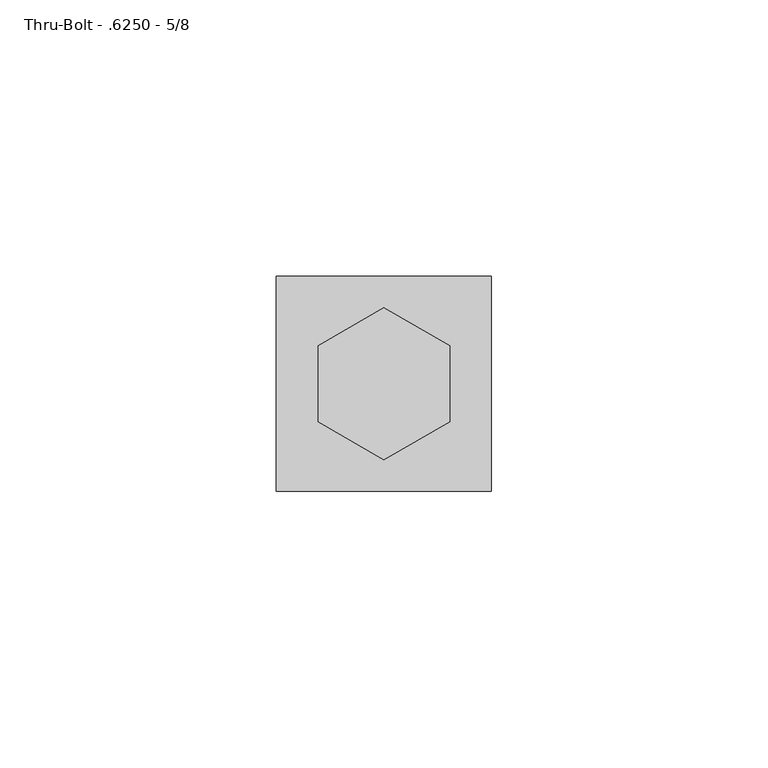
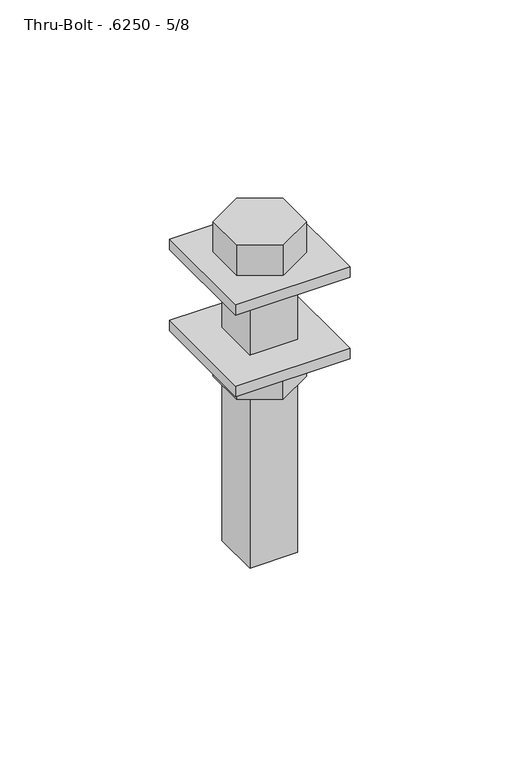
"""IFC4 building model written with IfcOpenShell, lengths in millimetres: fastener geometry, 060523 - W_P_C - Fastenings - Generic - SQUARE : Thru-Bolt - .6250 - 5/8."""

import ifcopenshell
import ifcopenshell.guid

model = None  # the IFC model being written
_history = None  # IfcOwnerHistory: only IFC2X3 demands one
_inside = {}  # id of a spatial element -> (the spatial element, [elements in it])
_under = {}  # id of a project, library or spatial element -> (it, [spatial elements below it])
_declared = {}  # id of a project -> (the project, [libraries it declares])
_typed = {}  # id of a type object -> (the type object, [elements of that type])
_made_of = {}  # id of a material, layer set ... -> (it, [elements and type objects made of it])


def new_model(schema):
    """Start an empty IFC model of exactly this schema.

    Asked for "IFC4X3", IfcOpenShell would pick the latest addendum, in which some entities
    have other attributes; the version numbers below select the first issue.
    IFC2X3 requires an IfcOwnerHistory on every rooted entity: one is made here for all.
    """
    global model, _history
    if schema == "IFC4X3":
        model = ifcopenshell.file(schema_version=(4, 3, 0, 0))
    else:
        model = ifcopenshell.file(schema=schema)
    _inside.clear()
    _under.clear()
    _declared.clear()
    _typed.clear()
    _made_of.clear()
    _history = None
    if model.schema == "IFC2X3":
        org = make("IfcOrganization", Name="unknown")
        user = make(
            "IfcPersonAndOrganization",
            ThePerson=make("IfcPerson", FamilyName="unknown"),
            TheOrganization=org,
        )
        app = make(
            "IfcApplication",
            ApplicationDeveloper=org,
            Version="unknown",
            ApplicationFullName="unknown",
            ApplicationIdentifier="unknown",
        )
        _history = make(
            "IfcOwnerHistory",
            OwningUser=user,
            OwningApplication=app,
            ChangeAction="ADDED",
            CreationDate=0,
        )
    return model


def make(cls, **values):
    """One entity of the class cls with the attributes given. An attribute that is None is left unset."""
    return model.create_entity(
        cls, **{name: value for name, value in values.items() if value is not None}
    )


def rooted(cls, **values):
    """An entity with a GlobalId (a new one), such as an element, a storey or a relation."""
    return make(cls, GlobalId=ifcopenshell.guid.new(), OwnerHistory=_history, **values)


def si_unit(unit_type, name, prefix=None):
    """IfcSIUnit, for example si_unit("LENGTHUNIT", "METRE", prefix="MILLI")."""
    return make("IfcSIUnit", UnitType=unit_type, Prefix=prefix, Name=name)


def assignment(units):
    """IfcUnitAssignment: the units of a project."""
    return None if units is None else make("IfcUnitAssignment", Units=units)


def point(xyz):
    """IfcCartesianPoint."""
    return None if xyz is None else make("IfcCartesianPoint", Coordinates=xyz)


def direction(xyz):
    """IfcDirection."""
    return None if xyz is None else make("IfcDirection", DirectionRatios=xyz)


def frame(location, z_axis=None, x_axis=None):
    """IfcAxis2Placement3D, a coordinate frame: its origin and axes. An axis left out is left unset."""
    return make(
        "IfcAxis2Placement3D",
        Location=point(location),
        Axis=direction(z_axis),
        RefDirection=direction(x_axis),
    )


def origin():
    """The frame at (0, 0, 0) with its axes left unset."""
    return frame((0.0, 0.0, 0.0))


def origin_with_axes():
    """The frame at (0, 0, 0) with the z axis (0, 0, 1) and the x axis (1, 0, 0) written out."""
    return frame((0.0, 0.0, 0.0), z_axis=(0.0, 0.0, 1.0), x_axis=(1.0, 0.0, 0.0))


def place(relative_to, where):
    """IfcLocalPlacement: puts the frame where relative to a parent placement (None: the world)."""
    return make(
        "IfcLocalPlacement", PlacementRelTo=relative_to, RelativePlacement=where
    )


def context(
    kind, dimensions, precision=None, world=None, true_north=None, identifier=None
):
    """IfcGeometricRepresentationContext, for example the 3D "Model" context."""
    return make(
        "IfcGeometricRepresentationContext",
        ContextIdentifier=identifier,
        ContextType=kind,
        CoordinateSpaceDimension=dimensions,
        Precision=precision,
        WorldCoordinateSystem=world,
        TrueNorth=true_north,
    )


def project(units=None, contexts=None):
    """IfcProject with its units and contexts."""
    return rooted(
        "IfcProject",
        Name="project",
        RepresentationContexts=contexts,
        UnitsInContext=assignment(units),
    )


def spatial(cls, under=None, at=None, **own):
    """A site, building, storey or space (cls), placed at a placement, below another one or the project."""
    s = rooted(cls, ObjectPlacement=at, **own)
    if under is not None:
        _under.setdefault(under.id(), (under, []))[1].append(s)
    return s


def polyline(points):
    """IfcPolyline through the points."""
    return make("IfcPolyline", Points=[point(p) for p in points])


def outline(outer, holes=None, kind="AREA"):
    """IfcArbitraryClosedProfileDef: a profile drawn as a closed curve; with holes, ...WithVoids."""
    if holes is None:
        return make("IfcArbitraryClosedProfileDef", ProfileType=kind, OuterCurve=outer)
    return make(
        "IfcArbitraryProfileDefWithVoids",
        ProfileType=kind,
        OuterCurve=outer,
        InnerCurves=holes,
    )


def extrude(swept, where, along, depth):
    """IfcExtrudedAreaSolid: the profile swept, set in the frame where, extruded along a direction by depth."""
    return make(
        "IfcExtrudedAreaSolid",
        SweptArea=swept,
        Position=where,
        ExtrudedDirection=direction(along),
        Depth=depth,
    )


def shape(context_of_items, identifier, shape_type, items):
    """IfcShapeRepresentation: the items that make up one representation, for example the "Body"."""
    return make(
        "IfcShapeRepresentation",
        ContextOfItems=context_of_items,
        RepresentationIdentifier=identifier,
        RepresentationType=shape_type,
        Items=items,
    )


def source(mapping_origin, context_of_items, identifier, shape_type, items):
    """IfcRepresentationMap: a shape defined once, which mapped items show again and again."""
    return make(
        "IfcRepresentationMap",
        MappingOrigin=mapping_origin,
        MappedRepresentation=shape(context_of_items, identifier, shape_type, items),
    )


def transform(
    local_origin,
    x_axis=None,
    y_axis=None,
    z_axis=None,
    scale=None,
    scale2=None,
    scale3=None,
    uniform=True,
):
    """IfcCartesianTransformationOperator3D, or its non-uniform kind. x_axis, y_axis, z_axis: its Axis1, 2, 3."""
    if uniform:
        return make(
            "IfcCartesianTransformationOperator3D",
            Axis1=direction(x_axis),
            Axis2=direction(y_axis),
            LocalOrigin=point(local_origin),
            Scale=scale,
            Axis3=direction(z_axis),
        )
    return make(
        "IfcCartesianTransformationOperator3DnonUniform",
        Axis1=direction(x_axis),
        Axis2=direction(y_axis),
        LocalOrigin=point(local_origin),
        Scale=scale,
        Axis3=direction(z_axis),
        Scale2=scale2,
        Scale3=scale3,
    )


def mapped(mapping_source, mapping_target):
    """IfcMappedItem: shows the shape of a source again, moved by a transform."""
    return make(
        "IfcMappedItem", MappingSource=mapping_source, MappingTarget=mapping_target
    )


def made_of(thing, what):
    """Note that an element or type object is made of a material, layer set ...; save() writes the relation."""
    if what is not None:
        _made_of.setdefault(what.id(), (what, []))[1].append(thing)
    return thing


def element(
    cls,
    number,
    at=None,
    inside=None,
    cuts=None,
    type_object=None,
    material=None,
    context=None,
    identifier="Body",
    shape_type=None,
    held_by="IfcProductDefinitionShape",
    body=None,
    shapes=None,
    **own,
):
    """One element of the class cls, such as IfcWall. Its Tag is "e" and its number.

    at: its placement. inside: the storey or other place that contains it. cuts: it is an
    opening in that element (IfcRelVoidsElement). A single representation is given by context,
    identifier, shape_type and body (its items); several are given by shapes. held_by: the class
    of the entity that holds the representations. save() writes the other relations.
    """
    e = rooted(cls, Tag="e%d" % number, ObjectPlacement=at, **own)
    if body is not None:
        shapes = [shape(context, identifier, shape_type, body)]
    if shapes is not None:
        e.Representation = make(held_by, Representations=shapes)
    if inside is not None:
        _inside.setdefault(inside.id(), (inside, []))[1].append(e)
    if cuts is not None:
        rooted(
            "IfcRelVoidsElement", RelatingBuildingElement=cuts, RelatedOpeningElement=e
        )
    if type_object is not None:
        _typed.setdefault(type_object.id(), (type_object, []))[1].append(e)
    return made_of(e, material)


def aggregate(whole, parts):
    """IfcRelAggregates: a whole, such as a stair, and the parts it consists of."""
    return rooted("IfcRelAggregates", RelatingObject=whole, RelatedObjects=parts)


def save(model, path):
    """Write the relations noted so far, then the file.

    IfcRelAggregates (storeys below a building ...), IfcRelContainedInSpatialStructure (elements
    in a storey), IfcRelDefinesByType, IfcRelAssociatesMaterial and IfcRelDeclares: one each for
    every whole, place, type object, material and project.
    """
    for whole, parts in _under.values():
        aggregate(whole, parts)
    for where, things in _inside.values():
        rooted(
            "IfcRelContainedInSpatialStructure",
            RelatedElements=things,
            RelatingStructure=where,
        )
    for kind, things in _typed.values():
        rooted("IfcRelDefinesByType", RelatedObjects=things, RelatingType=kind)
    for what, things in _made_of.values():
        rooted("IfcRelAssociatesMaterial", RelatedObjects=things, RelatingMaterial=what)
    for by, libraries in _declared.values():
        rooted("IfcRelDeclares", RelatingContext=by, RelatedDefinitions=libraries)
    model.write(path)


def thru_bolt_6250_5_8_f1e17e93(model_context):
    return source(origin(), model_context, "Body", "SweptSolid", [
        extrude(outline(polyline([(-19.446875, -19.446875), (-19.446875, 19.446875), (19.446875, 19.446875), (19.446875, -19.446875), (-19.446875, -19.446875)])), origin_with_axes(), (0.0, 0.0, 1.0), 3.7703125),
        extrude(outline(polyline([(-19.446875, -19.446875), (-19.446875, 19.446875), (19.446875, 19.446875), (19.446875, -19.446875), (-19.446875, -19.446875)])), frame((0.0, 0.0, -29.1703125), z_axis=(0.0, 0.0, 1.0), x_axis=(1.0, 0.0, 0.0)), (0.0, 0.0, 1.0), 3.7703125),
        extrude(outline(polyline([(-11.90625, -6.8740766), (-11.90625, 6.8740766), (0.0, 13.7481533), (11.90625, 6.8740766), (11.90625, -6.8740766), (0.0, -13.7481533), (-11.90625, -6.8740766)])), frame((0.0, 0.0, -40.48125), z_axis=(0.0, 0.0, 1.0), x_axis=(1.0, 0.0, 0.0)), (0.0, 0.0, 1.0), 11.3109375),
        extrude(outline(polyline([(-11.90625, 6.8740766), (0.0, 13.7481533), (11.90625, 6.8740766), (11.90625, -6.8740766), (0.0, -13.7481533), (-11.90625, -6.8740766), (-11.90625, 6.8740766)])), frame((0.0, 0.0, 3.7703125), z_axis=(0.0, 0.0, 1.0), x_axis=(1.0, 0.0, 0.0)), (0.0, 0.0, 1.0), 11.3109375),
        extrude(outline(polyline([(-8.1359375, 8.1359375), (8.1359375, 8.1359375), (8.1359375, -8.1359375), (-8.1359375, -8.1359375), (-8.1359375, 8.1359375)])), frame((0.0, 0.0, -101.6), z_axis=(0.0, 0.0, 1.0), x_axis=(1.0, 0.0, 0.0)), (0.0, 0.0, 1.0), 105.3703125),
    ])


if __name__ == "__main__":
    model = new_model("IFC4")
    model_context = context("Model", 3, world=origin())
    ifc_project = project(units=[si_unit("LENGTHUNIT", "METRE", prefix="MILLI")], contexts=[model_context])
    site = spatial("IfcSite", under=ifc_project)
    building = spatial("IfcBuilding", under=site)
    placement = place(None, origin())
    thru_bolt_6250_5_8_shape = thru_bolt_6250_5_8_f1e17e93(model_context)
    element("IfcFastener", 1, ObjectType="060523 - W_P_C - Fastenings - Generic - SQUARE : Thru-Bolt - .6250 - 5/8", at=placement, inside=building, context=model_context, shape_type="MappedRepresentation", body=[
        mapped(thru_bolt_6250_5_8_shape, transform((0.0, 0.0, 0.0), x_axis=(1.0, 0.0, 0.0), y_axis=(0.0, 1.0, 0.0), z_axis=(0.0, 0.0, 1.0))),
    ])
    save(model, "model.ifc")

# Revit data of these elements
# Type "060523 - W_P_C - Fastenings - Generic - SQUARE : Thru-Bolt - .6250 - 5/8"
#   Washer_Thickness = 0' - 0 19/128"
#   Washer Radius = 0' - 0 49/64"
#   Washer Offset - Head = 0' - 0 19/128"
#   Washer Offset = 0' - 0 19/128"
#   Thickness_of_Substrate [instance default] = 0' - 1"
#   Side = 0' - 0.54199"
#   Radius = 0' - 0 41/128"
#   Length [instance default] = 0' - 4"
#   Head Size = 0' - 0 15/16"
#   Head Radius = 0' - 0 15/32"
#   Head Height = 0' - 0 57/128"
#   Double Diameter = 0' - 1 9/32"
#   Diameter = 0' - 0 41/64"
#   Default Elevation = 4' - 0"
#   Washer_Nut_Visibility = yes
#   Washer_Head_Visibility = yes
#   Round_Head_Visibility = no
#   Point Visibility = no
#   Nut_Visibility = yes
#   Hex_Head_Visiblilty = yes
#   Washer Material = none
#   Bolt Material (Size) = AT SILL - FASTENER AT 24" O.C.
# Element 1 (IfcFastener, "060523 - W_P_C - Fastenings - Generic - SQUARE : Thru-Bolt - .6250 - 5/8")
#   Materials on its faces: "AT SILL - FASTENER AT 24\" O.C."
# Materials
#   "AT SILL - FASTENER AT 24\" O.C.": class "Generic", colour RGB 120 120 120, transparency 0, Cost = 0
